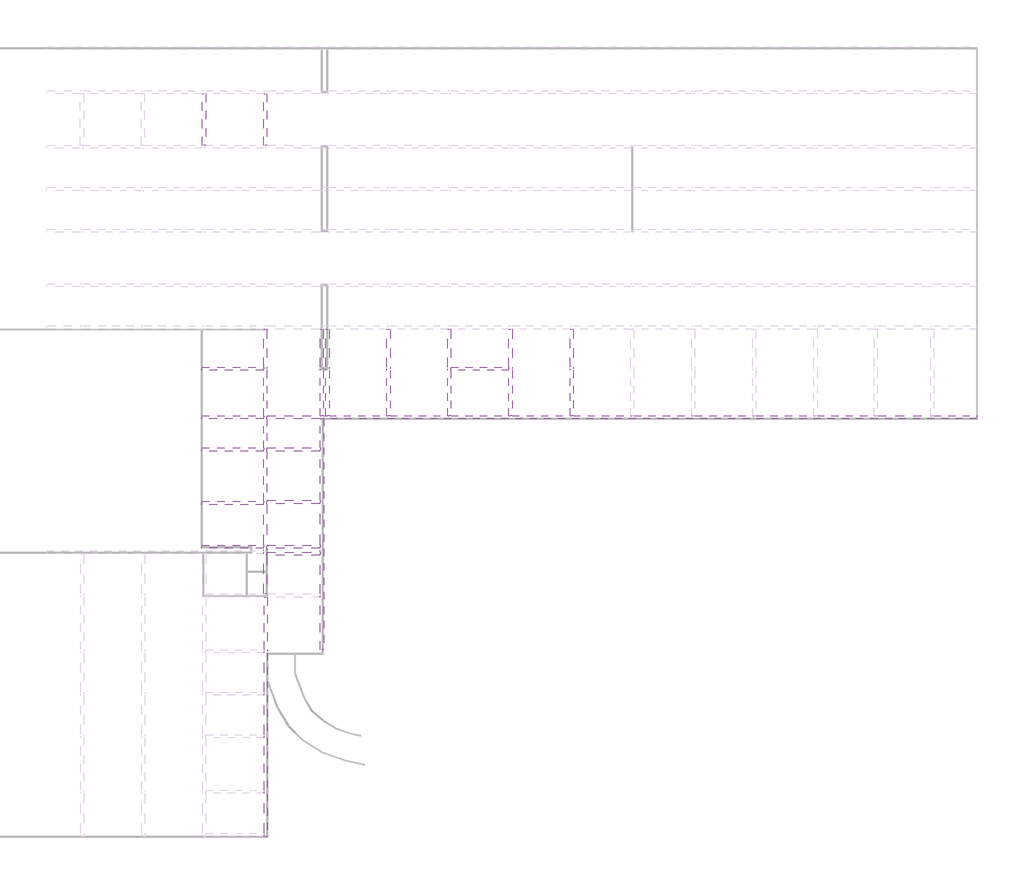
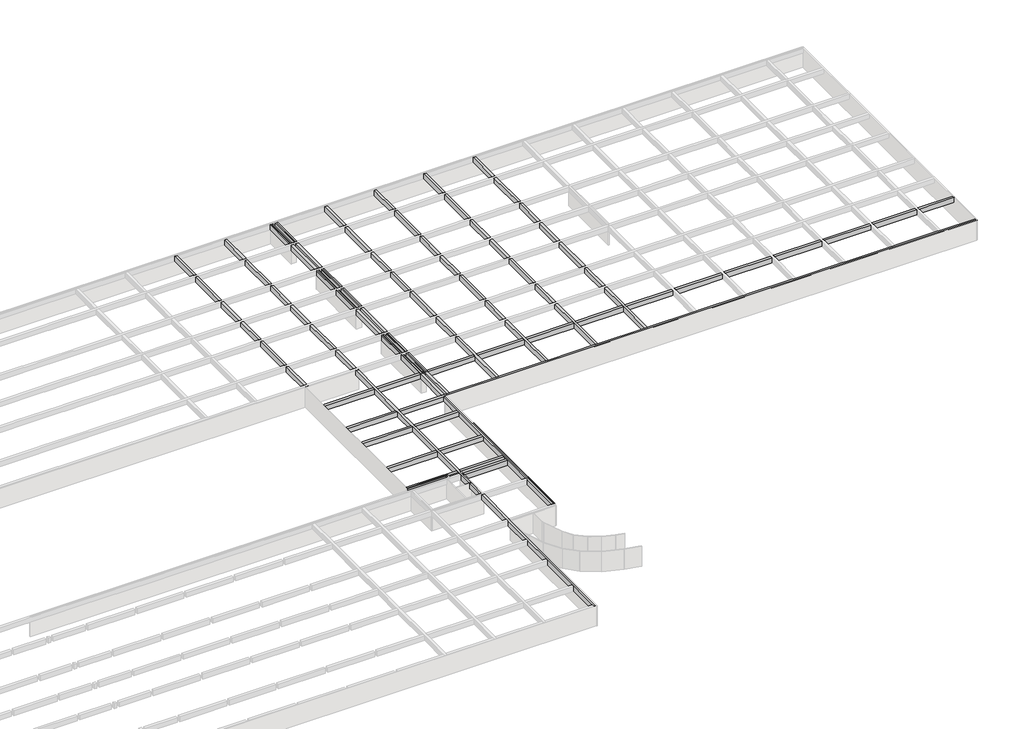
# One storey, part 13 of 14: 22 beams.
"""IFC4 building model written with IfcOpenShell, lengths in millimetres."""

from ifc_helpers import new_model, si_unit, frame, origin, place, context, project, spatial, polyline, outline, extrude, faceted_brep, element, save

model = new_model("IFC4")

# Units and contexts
model_context = context("Model", 3, world=origin())
ifc_project = project(units=[si_unit("LENGTHUNIT", "METRE", prefix="MILLI")], contexts=[model_context])

# Site, building, storey
site = spatial("IfcSite", under=ifc_project)
building = spatial("IfcBuilding", under=site)
storey = spatial("IfcBuildingStorey", under=building, Name="户型图", Elevation=0.0)

# Beams
placement = place(None, origin())
element("IfcBeam", 1, ObjectType="混凝土 - 矩形梁 : KL_beam", at=placement, inside=storey, context=model_context, shape_type="SweptSolid", body=[
    extrude(outline(polyline([(128527.2949044, -153358.950757), (128127.2949044, -153358.950757), (128127.2949044, -153299.284307), (128527.2949044, -153299.284307), (128527.2949044, -153358.950757)])), frame((0.0, 0.0, 2500.0), z_axis=(0.0, 0.0, 1.0), x_axis=(1.0, 0.0, 0.0)), (0.0, 0.0, 1.0), 800.0),
    extrude(outline(polyline([(128527.2949044, -122797.8127788), (128127.2949044, -122797.8127788), (128127.2949044, -117558.950757), (128527.2949044, -117558.950757), (128527.2949044, -122797.8127788)])), frame((0.0, 0.0, 2500.0), z_axis=(0.0, 0.0, 1.0), x_axis=(1.0, 0.0, 0.0)), (0.0, 0.0, 1.0), 800.0),
    extrude(outline(polyline([(128127.2949044, -123197.8127788), (128527.2949044, -123197.8127788), (128527.2949044, -129780.0179086), (128127.2949044, -129780.0179086), (128127.2949044, -123197.8127788)])), frame((0.0, 0.0, 2500.0), z_axis=(0.0, 0.0, 1.0), x_axis=(1.0, 0.0, 0.0)), (0.0, 0.0, 1.0), 800.0),
    extrude(outline(polyline([(128127.2949044, -130180.0179086), (128527.2949044, -130180.0179086), (128527.2949044, -135180.0179086), (128127.2949044, -135180.0179086), (128127.2949044, -130180.0179086)])), frame((0.0, 0.0, 2500.0), z_axis=(0.0, 0.0, 1.0), x_axis=(1.0, 0.0, 0.0)), (0.0, 0.0, 1.0), 800.0),
    extrude(outline(polyline([(128127.2949044, -135580.0179086), (128527.2949044, -135580.0179086), (128527.2949044, -140520.0179086), (128127.2949044, -140520.0179086), (128127.2949044, -135580.0179086)])), frame((0.0, 0.0, 2500.0), z_axis=(0.0, 0.0, 1.0), x_axis=(1.0, 0.0, 0.0)), (0.0, 0.0, 1.0), 800.0),
    extrude(outline(polyline([(128127.2949044, -140920.0179086), (128527.2949044, -140920.0179086), (128527.2949044, -147499.284307), (128127.2949044, -147499.284307), (128127.2949044, -140920.0179086)])), frame((0.0, 0.0, 2500.0), z_axis=(0.0, 0.0, 1.0), x_axis=(1.0, 0.0, 0.0)), (0.0, 0.0, 1.0), 800.0),
    extrude(outline(polyline([(128127.2949044, -147899.284307), (128527.2949044, -147899.284307), (128527.2949044, -152899.284307), (128127.2949044, -152899.284307), (128127.2949044, -147899.284307)])), frame((0.0, 0.0, 2500.0), z_axis=(0.0, 0.0, 1.0), x_axis=(1.0, 0.0, 0.0)), (0.0, 0.0, 1.0), 800.0),
])
element("IfcBeam", 2, ObjectType="混凝土 - 矩形梁 : KL_beam", at=placement, inside=storey, context=model_context, shape_type="SweptSolid", body=[
    extrude(outline(polyline([(136347.2949044, -153358.950757), (135947.2949044, -153358.950757), (135947.2949044, -153299.284307), (136347.2949044, -153299.284307), (136347.2949044, -153358.950757)])), frame((0.0, 0.0, 2500.0), z_axis=(0.0, 0.0, 1.0), x_axis=(1.0, 0.0, 0.0)), (0.0, 0.0, 1.0), 800.0),
    extrude(outline(polyline([(135947.2949044, -123197.8127788), (136347.2949044, -123197.8127788), (136347.2949044, -129780.0179086), (135947.2949044, -129780.0179086), (135947.2949044, -123197.8127788)])), frame((0.0, 0.0, 2500.0), z_axis=(0.0, 0.0, 1.0), x_axis=(1.0, 0.0, 0.0)), (0.0, 0.0, 1.0), 800.0),
    extrude(outline(polyline([(136347.2949044, -122797.8127788), (135947.2949044, -122797.8127788), (135947.2949044, -117558.950757), (136347.2949044, -117558.950757), (136347.2949044, -122797.8127788)])), frame((0.0, 0.0, 2500.0), z_axis=(0.0, 0.0, 1.0), x_axis=(1.0, 0.0, 0.0)), (0.0, 0.0, 1.0), 800.0),
    extrude(outline(polyline([(135947.2949044, -130180.0179086), (136347.2949044, -130180.0179086), (136347.2949044, -135180.0179086), (135947.2949044, -135180.0179086), (135947.2949044, -130180.0179086)])), frame((0.0, 0.0, 2500.0), z_axis=(0.0, 0.0, 1.0), x_axis=(1.0, 0.0, 0.0)), (0.0, 0.0, 1.0), 800.0),
    extrude(outline(polyline([(135947.2949044, -135580.0179086), (136347.2949044, -135580.0179086), (136347.2949044, -140520.0179086), (135947.2949044, -140520.0179086), (135947.2949044, -135580.0179086)])), frame((0.0, 0.0, 2500.0), z_axis=(0.0, 0.0, 1.0), x_axis=(1.0, 0.0, 0.0)), (0.0, 0.0, 1.0), 800.0),
    extrude(outline(polyline([(135947.2949044, -140920.0179086), (136347.2949044, -140920.0179086), (136347.2949044, -147499.284307), (135947.2949044, -147499.284307), (135947.2949044, -140920.0179086)])), frame((0.0, 0.0, 2500.0), z_axis=(0.0, 0.0, 1.0), x_axis=(1.0, 0.0, 0.0)), (0.0, 0.0, 1.0), 800.0),
    extrude(outline(polyline([(135947.2949044, -147899.284307), (136347.2949044, -147899.284307), (136347.2949044, -152899.284307), (135947.2949044, -152899.284307), (135947.2949044, -147899.284307)])), frame((0.0, 0.0, 2500.0), z_axis=(0.0, 0.0, 1.0), x_axis=(1.0, 0.0, 0.0)), (0.0, 0.0, 1.0), 800.0),
])
element("IfcBeam", 3, ObjectType="混凝土 - 矩形梁 : KL_beam", at=placement, inside=storey, context=model_context, shape_type="Brep", body=[
    faceted_brep([(143177.2949044, -122797.8127788, 3300.0), (143577.2949044, -122797.8127788, 3300.0), (143577.2949044, -117558.950757, 3300.0), (143177.2949044, -117558.950757, 3300.0), (143177.2949044, -122797.8127788, 2500.0), (143177.2949044, -117558.950757, 2500.0), (143577.2949044, -122797.8127788, 2500.0), (143577.2949044, -117558.950757, 2500.0)], [[[0, 1, 2, 3]], [[4, 0, 3, 5]], [[6, 4, 5, 7]], [[1, 6, 7, 2]], [[1, 0, 4, 6]], [[3, 2, 7, 5]]]),
    faceted_brep([(143177.2949044, -123197.8127788, 3300.0), (143577.2949044, -123197.8127788, 3300.0), (143577.2949044, -123197.8127788, 2500.0), (143177.2949044, -123197.8127788, 2500.0), (143577.2949044, -129780.0179086, 3300.0), (143177.2949044, -129780.0179086, 3300.0), (143177.2949044, -129780.0179086, 2500.0), (143577.2949044, -129780.0179086, 2500.0)], [[[0, 1, 2, 3]], [[4, 5, 6, 7]], [[1, 0, 5, 4]], [[0, 3, 6, 5]], [[3, 2, 7, 6]], [[2, 1, 4, 7]]]),
    faceted_brep([(143577.2949044, -130180.0179086, 3300.0), (143177.2949044, -130180.0179086, 3300.0), (143177.2949044, -135180.0179086, 3300.0), (143577.2949044, -135180.0179086, 3300.0), (143177.2949044, -130180.0179086, 2500.0), (143177.2949044, -135180.0179086, 2500.0), (143577.2949044, -130180.0179086, 2500.0), (143577.2949044, -135180.0179086, 2500.0)], [[[0, 1, 2, 3]], [[1, 4, 5, 2]], [[4, 6, 7, 5]], [[6, 0, 3, 7]], [[1, 0, 6, 4]], [[3, 2, 5, 7]]]),
    faceted_brep([(143177.2949044, -135580.0179086, 3300.0), (143577.2949044, -135580.0179086, 3300.0), (143577.2949044, -135580.0179086, 2500.0), (143177.2949044, -135580.0179086, 2500.0), (143577.2949044, -140520.0179086, 3300.0), (143177.2949044, -140520.0179086, 3300.0), (143177.2949044, -140520.0179086, 2500.0), (143577.2949044, -140520.0179086, 2500.0)], [[[0, 1, 2, 3]], [[4, 5, 6, 7]], [[1, 0, 5, 4]], [[0, 3, 6, 5]], [[3, 2, 7, 6]], [[2, 1, 4, 7]]]),
    faceted_brep([(143177.2949044, -140920.0179086, 3300.0), (143577.2949044, -140920.0179086, 3300.0), (143577.2949044, -140920.0179086, 2500.0), (143177.2949044, -140920.0179086, 2500.0), (143577.2949044, -147499.284307, 3300.0), (143177.2949044, -147499.284307, 3300.0), (143177.2949044, -147499.284307, 2500.0), (143577.2949044, -147499.284307, 2500.0)], [[[0, 1, 2, 3]], [[4, 5, 6, 7]], [[1, 0, 5, 4]], [[0, 3, 6, 5]], [[3, 2, 7, 6]], [[2, 1, 4, 7]]]),
    faceted_brep([(143177.2949044, -147899.284307, 3300.0), (143577.2949044, -147899.284307, 3300.0), (143577.2949044, -147899.284307, 2500.0), (143177.2949044, -147899.284307, 2500.0), (143577.2949044, -152899.284307, 3300.0), (143177.2949044, -152899.284307, 3300.0), (143177.2949044, -152899.284307, 2500.0), (143577.2949044, -152899.284307, 2500.0)], [[[0, 1, 2, 3]], [[4, 5, 6, 7]], [[1, 0, 5, 4]], [[0, 3, 6, 5]], [[3, 2, 7, 6]], [[2, 1, 4, 7]]]),
    faceted_brep([(143177.2949044, -153299.284307, 3300.0), (143577.2949044, -153299.284307, 3300.0), (143577.2949044, -153299.284307, 2500.0), (143177.2949044, -153299.284307, 2500.0), (143577.2949044, -164396.0449275, 3300.0), (143177.2949044, -164396.0449275, 3300.0), (143177.2949044, -164396.0449275, 2500.0), (143577.2949044, -164396.0449275, 2500.0), (143177.2949044, -158198.950757, 3300.0), (143177.2949044, -158598.950757, 3300.0), (143577.2949044, -158598.950757, 3300.0), (143577.2949044, -158198.950757, 3300.0), (143177.2949044, -158198.950757, 2500.0), (143177.2949044, -158598.950757, 2500.0), (143577.2949044, -158198.950757, 2500.0), (143577.2949044, -158598.950757, 2500.0)], [[[0, 1, 2, 3]], [[4, 5, 6, 7]], [[1, 0, 8, 9, 5, 4, 10, 11]], [[0, 3, 12, 13, 6, 5, 9, 8]], [[3, 2, 14, 15, 7, 6, 13, 12]], [[2, 1, 11, 10, 4, 7, 15, 14]]]),
])
element("IfcBeam", 4, ObjectType="混凝土 - 矩形梁 : KL_beam", at=placement, inside=storey, context=model_context, shape_type="Brep", body=[
    faceted_brep([(144337.2949044, -153299.284307, 3300.0), (143937.2949044, -153299.284307, 3300.0), (143937.2949044, -158198.950757, 3300.0), (143937.2949044, -158598.950757, 3300.0), (143937.2949044, -164396.0449275, 3300.0), (144337.2949044, -164396.0449275, 3300.0), (144337.2949044, -158598.950757, 3300.0), (144337.2949044, -158198.950757, 3300.0), (144337.2949044, -153299.284307, 2500.0), (144337.2949044, -164396.0449275, 2500.0), (144337.2949044, -158598.950757, 2500.0), (144337.2949044, -158198.950757, 2500.0), (143937.2949044, -153299.284307, 2500.0), (143937.2949044, -164396.0449275, 2500.0), (143937.2949044, -158598.950757, 2500.0), (143937.2949044, -158198.950757, 2500.0)], [[[0, 1, 2, 3, 4, 5, 6, 7]], [[8, 0, 7, 6, 5, 9, 10, 11]], [[12, 8, 11, 10, 9, 13, 14, 15]], [[1, 12, 15, 14, 13, 4, 3, 2]], [[1, 0, 8, 12]], [[5, 4, 13, 9]]]),
    faceted_brep([(143937.2949044, -123197.8127788, 3300.0), (144337.2949044, -123197.8127788, 3300.0), (144337.2949044, -123197.8127788, 2500.0), (143937.2949044, -123197.8127788, 2500.0), (144337.2949044, -129780.0179086, 3300.0), (143937.2949044, -129780.0179086, 3300.0), (143937.2949044, -129780.0179086, 2500.0), (144337.2949044, -129780.0179086, 2500.0)], [[[0, 1, 2, 3]], [[4, 5, 6, 7]], [[1, 0, 5, 4]], [[2, 1, 4, 7]], [[3, 2, 7, 6]], [[0, 3, 6, 5]]]),
    faceted_brep([(144337.2949044, -122797.8127788, 3300.0), (143937.2949044, -122797.8127788, 3300.0), (143937.2949044, -122797.8127788, 2500.0), (144337.2949044, -122797.8127788, 2500.0), (144337.2949044, -117558.950757, 3300.0), (143937.2949044, -117558.950757, 3300.0), (144337.2949044, -117558.950757, 2500.0), (143937.2949044, -117558.950757, 2500.0)], [[[0, 1, 2, 3]], [[1, 0, 4, 5]], [[0, 3, 6, 4]], [[3, 2, 7, 6]], [[2, 1, 5, 7]], [[5, 4, 6, 7]]]),
    faceted_brep([(143937.2949044, -130180.0179086, 3300.0), (144337.2949044, -130180.0179086, 3300.0), (144337.2949044, -130180.0179086, 2500.0), (143937.2949044, -130180.0179086, 2500.0), (144337.2949044, -135180.0179086, 3300.0), (143937.2949044, -135180.0179086, 3300.0), (143937.2949044, -135180.0179086, 2500.0), (144337.2949044, -135180.0179086, 2500.0)], [[[0, 1, 2, 3]], [[4, 5, 6, 7]], [[1, 0, 5, 4]], [[2, 1, 4, 7]], [[3, 2, 7, 6]], [[0, 3, 6, 5]]]),
    faceted_brep([(143937.2949044, -135580.0179086, 3300.0), (144337.2949044, -135580.0179086, 3300.0), (144337.2949044, -135580.0179086, 2500.0), (143937.2949044, -135580.0179086, 2500.0), (144337.2949044, -140520.0179086, 3300.0), (143937.2949044, -140520.0179086, 3300.0), (143937.2949044, -140520.0179086, 2500.0), (144337.2949044, -140520.0179086, 2500.0)], [[[0, 1, 2, 3]], [[4, 5, 6, 7]], [[1, 0, 5, 4]], [[2, 1, 4, 7]], [[3, 2, 7, 6]], [[0, 3, 6, 5]]]),
    faceted_brep([(143937.2949044, -140920.0179086, 3300.0), (144337.2949044, -140920.0179086, 3300.0), (144337.2949044, -140920.0179086, 2500.0), (143937.2949044, -140920.0179086, 2500.0), (144337.2949044, -147499.284307, 3300.0), (143937.2949044, -147499.284307, 3300.0), (143937.2949044, -147499.284307, 2500.0), (144337.2949044, -147499.284307, 2500.0)], [[[0, 1, 2, 3]], [[4, 5, 6, 7]], [[1, 0, 5, 4]], [[2, 1, 4, 7]], [[3, 2, 7, 6]], [[0, 3, 6, 5]]]),
    faceted_brep([(143937.2949044, -147899.284307, 3300.0), (144337.2949044, -147899.284307, 3300.0), (144337.2949044, -147899.284307, 2500.0), (143937.2949044, -147899.284307, 2500.0), (144337.2949044, -152899.284307, 3300.0), (143937.2949044, -152899.284307, 3300.0), (143937.2949044, -152899.284307, 2500.0), (144337.2949044, -152899.284307, 2500.0)], [[[0, 1, 2, 3]], [[4, 5, 6, 7]], [[1, 0, 5, 4]], [[2, 1, 4, 7]], [[3, 2, 7, 6]], [[0, 3, 6, 5]]]),
])
element("IfcBeam", 5, ObjectType="混凝土 - 矩形梁 : KL_beam", at=placement, inside=storey, context=model_context, shape_type="Brep", body=[
    faceted_brep([(151740.9658811, -122797.8127788, 3300.0), (152140.9658811, -122797.8127788, 3300.0), (152140.9658811, -117558.950757, 3300.0), (151740.9658811, -117558.950757, 3300.0), (151740.9658811, -122797.8127788, 2500.0), (151740.9658811, -117558.950757, 2500.0), (152140.9658811, -122797.8127788, 2500.0), (152140.9658811, -117558.950757, 2500.0)], [[[0, 1, 2, 3]], [[4, 0, 3, 5]], [[6, 4, 5, 7]], [[1, 6, 7, 2]], [[1, 0, 4, 6]], [[3, 2, 7, 5]]]),
    faceted_brep([(151740.9658811, -123197.8127788, 3300.0), (152140.9658811, -123197.8127788, 3300.0), (152140.9658811, -123197.8127788, 2500.0), (151740.9658811, -123197.8127788, 2500.0), (152140.9658811, -129780.0179086, 3300.0), (151740.9658811, -129780.0179086, 3300.0), (151740.9658811, -129780.0179086, 2500.0), (152140.9658811, -129780.0179086, 2500.0)], [[[0, 1, 2, 3]], [[4, 5, 6, 7]], [[1, 0, 5, 4]], [[0, 3, 6, 5]], [[3, 2, 7, 6]], [[2, 1, 4, 7]]]),
    faceted_brep([(152140.9658811, -130180.0179086, 3300.0), (151740.9658811, -130180.0179086, 3300.0), (151740.9658811, -135180.0179086, 3300.0), (152140.9658811, -135180.0179086, 3300.0), (151740.9658811, -130180.0179086, 2500.0), (151740.9658811, -135180.0179086, 2500.0), (152140.9658811, -130180.0179086, 2500.0), (152140.9658811, -135180.0179086, 2500.0)], [[[0, 1, 2, 3]], [[1, 4, 5, 2]], [[4, 6, 7, 5]], [[6, 0, 3, 7]], [[1, 0, 6, 4]], [[3, 2, 5, 7]]]),
    faceted_brep([(151740.9658811, -135580.0179086, 3300.0), (152140.9658811, -135580.0179086, 3300.0), (152140.9658811, -135580.0179086, 2500.0), (151740.9658811, -135580.0179086, 2500.0), (152140.9658811, -140520.0179086, 3300.0), (151740.9658811, -140520.0179086, 3300.0), (151740.9658811, -140520.0179086, 2500.0), (152140.9658811, -140520.0179086, 2500.0)], [[[0, 1, 2, 3]], [[4, 5, 6, 7]], [[1, 0, 5, 4]], [[0, 3, 6, 5]], [[3, 2, 7, 6]], [[2, 1, 4, 7]]]),
    faceted_brep([(151740.9658811, -140920.0179086, 3300.0), (152140.9658811, -140920.0179086, 3300.0), (152140.9658811, -140920.0179086, 2500.0), (151740.9658811, -140920.0179086, 2500.0), (152140.9658811, -147499.284307, 3300.0), (151740.9658811, -147499.284307, 3300.0), (151740.9658811, -147499.284307, 2500.0), (152140.9658811, -147499.284307, 2500.0)], [[[0, 1, 2, 3]], [[4, 5, 6, 7]], [[1, 0, 5, 4]], [[0, 3, 6, 5]], [[3, 2, 7, 6]], [[2, 1, 4, 7]]]),
    faceted_brep([(151740.9658811, -147899.284307, 3300.0), (152140.9658811, -147899.284307, 3300.0), (152140.9658811, -147899.284307, 2500.0), (151740.9658811, -147899.284307, 2500.0), (152140.9658811, -152899.284307, 3300.0), (151740.9658811, -152899.284307, 3300.0), (151740.9658811, -152899.284307, 2500.0), (152140.9658811, -152899.284307, 2500.0)], [[[0, 1, 2, 3]], [[4, 5, 6, 7]], [[1, 0, 5, 4]], [[0, 3, 6, 5]], [[3, 2, 7, 6]], [[2, 1, 4, 7]]]),
    faceted_brep([(151740.9658811, -153299.284307, 3300.0), (152140.9658811, -153299.284307, 3300.0), (152140.9658811, -153299.284307, 2500.0), (151740.9658811, -153299.284307, 2500.0), (152140.9658811, -164396.0449275, 3300.0), (151740.9658811, -164396.0449275, 3300.0), (151740.9658811, -164396.0449275, 2500.0), (152140.9658811, -164396.0449275, 2500.0), (151740.9658811, -158198.950757, 3300.0), (151740.9658811, -158598.950757, 3300.0), (152140.9658811, -158598.950757, 3300.0), (152140.9658811, -158198.950757, 3300.0), (151740.9658811, -158198.950757, 2500.0), (151740.9658811, -158598.950757, 2500.0), (152140.9658811, -158198.950757, 2500.0), (152140.9658811, -158598.950757, 2500.0)], [[[0, 1, 2, 3]], [[4, 5, 6, 7]], [[1, 0, 8, 9, 5, 4, 10, 11]], [[0, 3, 12, 13, 6, 5, 9, 8]], [[3, 2, 14, 15, 7, 6, 13, 12]], [[2, 1, 11, 10, 4, 7, 15, 14]]]),
])
element("IfcBeam", 6, ObjectType="混凝土 - 矩形梁 : KL_beam", at=placement, inside=storey, context=model_context, shape_type="Brep", body=[
    faceted_brep([(159907.8874304, -153299.284307, 3300.0), (159507.8874304, -153299.284307, 3300.0), (159507.8874304, -158198.950757, 3300.0), (159507.8874304, -158598.950757, 3300.0), (159507.8874304, -164396.0449275, 3300.0), (159907.8874304, -164396.0449275, 3300.0), (159907.8874304, -158598.950757, 3300.0), (159907.8874304, -158198.950757, 3300.0), (159907.8874304, -153299.284307, 2500.0), (159907.8874304, -164396.0449275, 2500.0), (159907.8874304, -158598.950757, 2500.0), (159907.8874304, -158198.950757, 2500.0), (159507.8874304, -153299.284307, 2500.0), (159507.8874304, -164396.0449275, 2500.0), (159507.8874304, -158598.950757, 2500.0), (159507.8874304, -158198.950757, 2500.0)], [[[0, 1, 2, 3, 4, 5, 6, 7]], [[8, 0, 7, 6, 5, 9, 10, 11]], [[12, 8, 11, 10, 9, 13, 14, 15]], [[1, 12, 15, 14, 13, 4, 3, 2]], [[1, 0, 8, 12]], [[5, 4, 13, 9]]]),
    faceted_brep([(159507.8874304, -123197.8127788, 3300.0), (159907.8874304, -123197.8127788, 3300.0), (159907.8874304, -123197.8127788, 2500.0), (159507.8874304, -123197.8127788, 2500.0), (159907.8874304, -129780.0179086, 3300.0), (159507.8874304, -129780.0179086, 3300.0), (159507.8874304, -129780.0179086, 2500.0), (159907.8874304, -129780.0179086, 2500.0)], [[[0, 1, 2, 3]], [[4, 5, 6, 7]], [[1, 0, 5, 4]], [[2, 1, 4, 7]], [[3, 2, 7, 6]], [[0, 3, 6, 5]]]),
    faceted_brep([(159907.8874304, -122797.8127788, 3300.0), (159507.8874304, -122797.8127788, 3300.0), (159507.8874304, -122797.8127788, 2500.0), (159907.8874304, -122797.8127788, 2500.0), (159907.8874304, -117558.950757, 3300.0), (159507.8874304, -117558.950757, 3300.0), (159907.8874304, -117558.950757, 2500.0), (159507.8874304, -117558.950757, 2500.0)], [[[0, 1, 2, 3]], [[1, 0, 4, 5]], [[0, 3, 6, 4]], [[3, 2, 7, 6]], [[2, 1, 5, 7]], [[5, 4, 6, 7]]]),
    faceted_brep([(159507.8874304, -130180.0179086, 3300.0), (159907.8874304, -130180.0179086, 3300.0), (159907.8874304, -130180.0179086, 2500.0), (159507.8874304, -130180.0179086, 2500.0), (159907.8874304, -135180.0179086, 3300.0), (159507.8874304, -135180.0179086, 3300.0), (159507.8874304, -135180.0179086, 2500.0), (159907.8874304, -135180.0179086, 2500.0)], [[[0, 1, 2, 3]], [[4, 5, 6, 7]], [[1, 0, 5, 4]], [[2, 1, 4, 7]], [[3, 2, 7, 6]], [[0, 3, 6, 5]]]),
    faceted_brep([(159507.8874304, -135580.0179086, 3300.0), (159907.8874304, -135580.0179086, 3300.0), (159907.8874304, -135580.0179086, 2500.0), (159507.8874304, -135580.0179086, 2500.0), (159907.8874304, -140520.0179086, 3300.0), (159507.8874304, -140520.0179086, 3300.0), (159507.8874304, -140520.0179086, 2500.0), (159907.8874304, -140520.0179086, 2500.0)], [[[0, 1, 2, 3]], [[4, 5, 6, 7]], [[1, 0, 5, 4]], [[2, 1, 4, 7]], [[3, 2, 7, 6]], [[0, 3, 6, 5]]]),
    faceted_brep([(159507.8874304, -140920.0179086, 3300.0), (159907.8874304, -140920.0179086, 3300.0), (159907.8874304, -140920.0179086, 2500.0), (159507.8874304, -140920.0179086, 2500.0), (159907.8874304, -147499.284307, 3300.0), (159507.8874304, -147499.284307, 3300.0), (159507.8874304, -147499.284307, 2500.0), (159907.8874304, -147499.284307, 2500.0)], [[[0, 1, 2, 3]], [[4, 5, 6, 7]], [[1, 0, 5, 4]], [[2, 1, 4, 7]], [[3, 2, 7, 6]], [[0, 3, 6, 5]]]),
    faceted_brep([(159507.8874304, -147899.284307, 3300.0), (159907.8874304, -147899.284307, 3300.0), (159907.8874304, -147899.284307, 2500.0), (159507.8874304, -147899.284307, 2500.0), (159907.8874304, -152899.284307, 3300.0), (159507.8874304, -152899.284307, 3300.0), (159507.8874304, -152899.284307, 2500.0), (159907.8874304, -152899.284307, 2500.0)], [[[0, 1, 2, 3]], [[4, 5, 6, 7]], [[1, 0, 5, 4]], [[2, 1, 4, 7]], [[3, 2, 7, 6]], [[0, 3, 6, 5]]]),
])
element("IfcBeam", 7, ObjectType="混凝土 - 矩形梁 : KL_beam", at=placement, inside=storey, context=model_context, shape_type="Brep", body=[
    faceted_brep([(167340.9658811, -122797.8127788, 3300.0), (167740.9658811, -122797.8127788, 3300.0), (167740.9658811, -117558.950757, 3300.0), (167340.9658811, -117558.950757, 3300.0), (167340.9658811, -122797.8127788, 2500.0), (167340.9658811, -117558.950757, 2500.0), (167740.9658811, -122797.8127788, 2500.0), (167740.9658811, -117558.950757, 2500.0)], [[[0, 1, 2, 3]], [[4, 0, 3, 5]], [[6, 4, 5, 7]], [[1, 6, 7, 2]], [[1, 0, 4, 6]], [[3, 2, 7, 5]]]),
    faceted_brep([(167340.9658811, -123197.8127788, 3300.0), (167740.9658811, -123197.8127788, 3300.0), (167740.9658811, -123197.8127788, 2500.0), (167340.9658811, -123197.8127788, 2500.0), (167740.9658811, -129780.0179086, 3300.0), (167340.9658811, -129780.0179086, 3300.0), (167340.9658811, -129780.0179086, 2500.0), (167740.9658811, -129780.0179086, 2500.0)], [[[0, 1, 2, 3]], [[4, 5, 6, 7]], [[1, 0, 5, 4]], [[0, 3, 6, 5]], [[3, 2, 7, 6]], [[2, 1, 4, 7]]]),
    faceted_brep([(167740.9658811, -130180.0179086, 3300.0), (167340.9658811, -130180.0179086, 3300.0), (167340.9658811, -135180.0179086, 3300.0), (167740.9658811, -135180.0179086, 3300.0), (167340.9658811, -130180.0179086, 2500.0), (167340.9658811, -135180.0179086, 2500.0), (167740.9658811, -130180.0179086, 2500.0), (167740.9658811, -135180.0179086, 2500.0)], [[[0, 1, 2, 3]], [[1, 4, 5, 2]], [[4, 6, 7, 5]], [[6, 0, 3, 7]], [[1, 0, 6, 4]], [[3, 2, 5, 7]]]),
    faceted_brep([(167340.9658811, -135580.0179086, 3300.0), (167740.9658811, -135580.0179086, 3300.0), (167740.9658811, -135580.0179086, 2500.0), (167340.9658811, -135580.0179086, 2500.0), (167740.9658811, -140520.0179086, 3300.0), (167340.9658811, -140520.0179086, 3300.0), (167340.9658811, -140520.0179086, 2500.0), (167740.9658811, -140520.0179086, 2500.0)], [[[0, 1, 2, 3]], [[4, 5, 6, 7]], [[1, 0, 5, 4]], [[0, 3, 6, 5]], [[3, 2, 7, 6]], [[2, 1, 4, 7]]]),
    faceted_brep([(167340.9658811, -140920.0179086, 3300.0), (167740.9658811, -140920.0179086, 3300.0), (167740.9658811, -140920.0179086, 2500.0), (167340.9658811, -140920.0179086, 2500.0), (167740.9658811, -147499.284307, 3300.0), (167340.9658811, -147499.284307, 3300.0), (167340.9658811, -147499.284307, 2500.0), (167740.9658811, -147499.284307, 2500.0)], [[[0, 1, 2, 3]], [[4, 5, 6, 7]], [[1, 0, 5, 4]], [[0, 3, 6, 5]], [[3, 2, 7, 6]], [[2, 1, 4, 7]]]),
    faceted_brep([(167340.9658811, -147899.284307, 3300.0), (167740.9658811, -147899.284307, 3300.0), (167740.9658811, -147899.284307, 2500.0), (167340.9658811, -147899.284307, 2500.0), (167740.9658811, -152899.284307, 3300.0), (167340.9658811, -152899.284307, 3300.0), (167340.9658811, -152899.284307, 2500.0), (167740.9658811, -152899.284307, 2500.0)], [[[0, 1, 2, 3]], [[4, 5, 6, 7]], [[1, 0, 5, 4]], [[0, 3, 6, 5]], [[3, 2, 7, 6]], [[2, 1, 4, 7]]]),
    faceted_brep([(167340.9658811, -153299.284307, 3300.0), (167740.9658811, -153299.284307, 3300.0), (167740.9658811, -153299.284307, 2500.0), (167340.9658811, -153299.284307, 2500.0), (167740.9658811, -164396.0449275, 3300.0), (167340.9658811, -164396.0449275, 3300.0), (167340.9658811, -164396.0449275, 2500.0), (167740.9658811, -164396.0449275, 2500.0), (167340.9658811, -158198.950757, 3300.0), (167340.9658811, -158598.950757, 3300.0), (167740.9658811, -158598.950757, 3300.0), (167740.9658811, -158198.950757, 3300.0), (167340.9658811, -158198.950757, 2500.0), (167340.9658811, -158598.950757, 2500.0), (167740.9658811, -158198.950757, 2500.0), (167740.9658811, -158598.950757, 2500.0)], [[[0, 1, 2, 3]], [[4, 5, 6, 7]], [[1, 0, 8, 9, 5, 4, 10, 11]], [[0, 3, 12, 13, 6, 5, 9, 8]], [[3, 2, 14, 15, 7, 6, 13, 12]], [[2, 1, 11, 10, 4, 7, 15, 14]]]),
])
element("IfcBeam", 8, ObjectType="混凝土 - 矩形梁 : KL_beam", at=placement, inside=storey, context=model_context, shape_type="Brep", body=[
    faceted_brep([(175558.5232577, -153299.284307, 3300.0), (175158.5232577, -153299.284307, 3300.0), (175158.5232577, -158198.950757, 3300.0), (175158.5232577, -158598.950757, 3300.0), (175158.5232577, -164396.0449275, 3300.0), (175558.5232577, -164396.0449275, 3300.0), (175558.5232577, -158598.950757, 3300.0), (175558.5232577, -158198.950757, 3300.0), (175558.5232577, -153299.284307, 2500.0), (175558.5232577, -164396.0449275, 2500.0), (175558.5232577, -158598.950757, 2500.0), (175558.5232577, -158198.950757, 2500.0), (175158.5232577, -153299.284307, 2500.0), (175158.5232577, -164396.0449275, 2500.0), (175158.5232577, -158598.950757, 2500.0), (175158.5232577, -158198.950757, 2500.0)], [[[0, 1, 2, 3, 4, 5, 6, 7]], [[8, 0, 7, 6, 5, 9, 10, 11]], [[12, 8, 11, 10, 9, 13, 14, 15]], [[1, 12, 15, 14, 13, 4, 3, 2]], [[1, 0, 8, 12]], [[5, 4, 13, 9]]]),
    faceted_brep([(175158.5232577, -123197.8127788, 3300.0), (175558.5232577, -123197.8127788, 3300.0), (175558.5232577, -123197.8127788, 2500.0), (175158.5232577, -123197.8127788, 2500.0), (175558.5232577, -129780.0179086, 3300.0), (175158.5232577, -129780.0179086, 3300.0), (175158.5232577, -129780.0179086, 2500.0), (175558.5232577, -129780.0179086, 2500.0)], [[[0, 1, 2, 3]], [[4, 5, 6, 7]], [[1, 0, 5, 4]], [[2, 1, 4, 7]], [[3, 2, 7, 6]], [[0, 3, 6, 5]]]),
    faceted_brep([(175558.5232577, -122797.8127788, 3300.0), (175158.5232577, -122797.8127788, 3300.0), (175158.5232577, -122797.8127788, 2500.0), (175558.5232577, -122797.8127788, 2500.0), (175558.5232577, -117558.950757, 3300.0), (175158.5232577, -117558.950757, 3300.0), (175558.5232577, -117558.950757, 2500.0), (175158.5232577, -117558.950757, 2500.0)], [[[0, 1, 2, 3]], [[1, 0, 4, 5]], [[0, 3, 6, 4]], [[3, 2, 7, 6]], [[2, 1, 5, 7]], [[5, 4, 6, 7]]]),
    faceted_brep([(175158.5232577, -130180.0179086, 3300.0), (175558.5232577, -130180.0179086, 3300.0), (175558.5232577, -130180.0179086, 2500.0), (175158.5232577, -130180.0179086, 2500.0), (175558.5232577, -135180.0179086, 3300.0), (175158.5232577, -135180.0179086, 3300.0), (175158.5232577, -135180.0179086, 2500.0), (175558.5232577, -135180.0179086, 2500.0)], [[[0, 1, 2, 3]], [[4, 5, 6, 7]], [[1, 0, 5, 4]], [[2, 1, 4, 7]], [[3, 2, 7, 6]], [[0, 3, 6, 5]]]),
    faceted_brep([(175158.5232577, -135580.0179086, 3300.0), (175558.5232577, -135580.0179086, 3300.0), (175558.5232577, -135580.0179086, 2500.0), (175158.5232577, -135580.0179086, 2500.0), (175558.5232577, -140520.0179086, 3300.0), (175158.5232577, -140520.0179086, 3300.0), (175158.5232577, -140520.0179086, 2500.0), (175558.5232577, -140520.0179086, 2500.0)], [[[0, 1, 2, 3]], [[4, 5, 6, 7]], [[1, 0, 5, 4]], [[2, 1, 4, 7]], [[3, 2, 7, 6]], [[0, 3, 6, 5]]]),
    faceted_brep([(175158.5232577, -140920.0179086, 3300.0), (175558.5232577, -140920.0179086, 3300.0), (175558.5232577, -140920.0179086, 2500.0), (175158.5232577, -140920.0179086, 2500.0), (175558.5232577, -147499.284307, 3300.0), (175158.5232577, -147499.284307, 3300.0), (175158.5232577, -147499.284307, 2500.0), (175558.5232577, -147499.284307, 2500.0)], [[[0, 1, 2, 3]], [[4, 5, 6, 7]], [[1, 0, 5, 4]], [[2, 1, 4, 7]], [[3, 2, 7, 6]], [[0, 3, 6, 5]]]),
    faceted_brep([(175158.5232577, -147899.284307, 3300.0), (175558.5232577, -147899.284307, 3300.0), (175558.5232577, -147899.284307, 2500.0), (175158.5232577, -147899.284307, 2500.0), (175558.5232577, -152899.284307, 3300.0), (175158.5232577, -152899.284307, 3300.0), (175158.5232577, -152899.284307, 2500.0), (175558.5232577, -152899.284307, 2500.0)], [[[0, 1, 2, 3]], [[4, 5, 6, 7]], [[1, 0, 5, 4]], [[2, 1, 4, 7]], [[3, 2, 7, 6]], [[0, 3, 6, 5]]]),
])
element("IfcBeam", 9, ObjectType="混凝土 - 矩形梁 : KL_beam", at=placement, inside=storey, context=model_context, shape_type="SweptSolid", body=[
    extrude(outline(polyline([(227227.2949044, -158198.950757), (227227.2949044, -158598.950757), (221727.2949044, -158598.950757), (221727.2949044, -158198.950757), (227227.2949044, -158198.950757)])), frame((0.0, 0.0, 2500.0), z_axis=(0.0, 0.0, 1.0), x_axis=(1.0, 0.0, 0.0)), (0.0, 0.0, 1.0), 800.0),
    extrude(outline(polyline([(143177.2949044, -158198.950757), (143177.2949044, -158598.950757), (136347.2949044, -158598.950757), (136347.2949044, -158198.950757), (143177.2949044, -158198.950757)])), frame((0.0, 0.0, 2500.0), z_axis=(0.0, 0.0, 1.0), x_axis=(1.0, 0.0, 0.0)), (0.0, 0.0, 1.0), 800.0),
    extrude(outline(polyline([(143577.2949044, -158598.950757), (143577.2949044, -158198.950757), (143937.2949044, -158198.950757), (143937.2949044, -158598.950757), (143577.2949044, -158598.950757)])), frame((0.0, 0.0, 2500.0), z_axis=(0.0, 0.0, 1.0), x_axis=(1.0, 0.0, 0.0)), (0.0, 0.0, 1.0), 800.0),
    extrude(outline(polyline([(144337.2949044, -158598.950757), (144337.2949044, -158198.950757), (151740.9658811, -158198.950757), (151740.9658811, -158598.950757), (144337.2949044, -158598.950757)])), frame((0.0, 0.0, 2500.0), z_axis=(0.0, 0.0, 1.0), x_axis=(1.0, 0.0, 0.0)), (0.0, 0.0, 1.0), 800.0),
    extrude(outline(polyline([(152140.9658811, -158598.950757), (152140.9658811, -158198.950757), (159507.8874304, -158198.950757), (159507.8874304, -158598.950757), (152140.9658811, -158598.950757)])), frame((0.0, 0.0, 2500.0), z_axis=(0.0, 0.0, 1.0), x_axis=(1.0, 0.0, 0.0)), (0.0, 0.0, 1.0), 800.0),
    extrude(outline(polyline([(159907.8874304, -158598.950757), (159907.8874304, -158198.950757), (167340.9658811, -158198.950757), (167340.9658811, -158598.950757), (159907.8874304, -158598.950757)])), frame((0.0, 0.0, 2500.0), z_axis=(0.0, 0.0, 1.0), x_axis=(1.0, 0.0, 0.0)), (0.0, 0.0, 1.0), 800.0),
    extrude(outline(polyline([(167740.9658811, -158598.950757), (167740.9658811, -158198.950757), (175158.5232577, -158198.950757), (175158.5232577, -158598.950757), (167740.9658811, -158598.950757)])), frame((0.0, 0.0, 2500.0), z_axis=(0.0, 0.0, 1.0), x_axis=(1.0, 0.0, 0.0)), (0.0, 0.0, 1.0), 800.0),
    extrude(outline(polyline([(175558.5232577, -158598.950757), (175558.5232577, -158198.950757), (182927.7006088, -158198.950757), (182927.7006088, -158598.950757), (175558.5232577, -158598.950757)])), frame((0.0, 0.0, 2500.0), z_axis=(0.0, 0.0, 1.0), x_axis=(1.0, 0.0, 0.0)), (0.0, 0.0, 1.0), 800.0),
    extrude(outline(polyline([(183327.7006088, -158598.950757), (183327.7006088, -158198.950757), (190737.2949044, -158198.950757), (190737.2949044, -158598.950757), (183327.7006088, -158598.950757)])), frame((0.0, 0.0, 2500.0), z_axis=(0.0, 0.0, 1.0), x_axis=(1.0, 0.0, 0.0)), (0.0, 0.0, 1.0), 800.0),
    extrude(outline(polyline([(191137.2949044, -158598.950757), (191137.2949044, -158198.950757), (198549.6658892, -158198.950757), (198549.6658892, -158598.950757), (191137.2949044, -158598.950757)])), frame((0.0, 0.0, 2500.0), z_axis=(0.0, 0.0, 1.0), x_axis=(1.0, 0.0, 0.0)), (0.0, 0.0, 1.0), 800.0),
    extrude(outline(polyline([(198949.6658892, -158598.950757), (198949.6658892, -158198.950757), (206363.3308695, -158198.950757), (206363.3308695, -158598.950757), (198949.6658892, -158598.950757)])), frame((0.0, 0.0, 2500.0), z_axis=(0.0, 0.0, 1.0), x_axis=(1.0, 0.0, 0.0)), (0.0, 0.0, 1.0), 800.0),
    extrude(outline(polyline([(206763.3308695, -158598.950757), (206763.3308695, -158198.950757), (214091.1566028, -158198.950757), (214091.1566028, -158598.950757), (206763.3308695, -158598.950757)])), frame((0.0, 0.0, 2500.0), z_axis=(0.0, 0.0, 1.0), x_axis=(1.0, 0.0, 0.0)), (0.0, 0.0, 1.0), 800.0),
    extrude(outline(polyline([(214491.1566028, -158598.950757), (214491.1566028, -158198.950757), (221327.2949044, -158198.950757), (221327.2949044, -158598.950757), (214491.1566028, -158598.950757)])), frame((0.0, 0.0, 2500.0), z_axis=(0.0, 0.0, 1.0), x_axis=(1.0, 0.0, 0.0)), (0.0, 0.0, 1.0), 800.0),
])
element("IfcBeam", 10, ObjectType="混凝土 - 矩形梁 : KL_beam", at=placement, inside=storey, context=model_context, shape_type="Brep", body=[
    faceted_brep([(136347.2949044, -153358.950757, 3300.0), (135947.2949044, -153358.950757, 3300.0), (135947.2949044, -158198.950757, 3300.0), (135947.2949044, -158598.950757, 3300.0), (135947.2949044, -164396.0449275, 3300.0), (135947.2949044, -164796.0449275, 3300.0), (135947.2949044, -168516.0449275, 3300.0), (135947.2949044, -168916.0449275, 3300.0), (135947.2949044, -175355.5769678, 3300.0), (135947.2949044, -175755.5769678, 3300.0), (135947.2949044, -180948.950757, 3300.0), (135947.2949044, -181348.950757, 3300.0), (135947.2949044, -181668.950757, 3300.0), (135947.2949044, -182068.950757, 3300.0), (135947.2949044, -187198.950757, 3300.0), (136347.2949044, -187198.950757, 3300.0), (136347.2949044, -182268.950757, 3300.0), (136347.2949044, -181868.950757, 3300.0), (136347.2949044, -181348.950757, 3300.0), (136347.2949044, -180948.950757, 3300.0), (136347.2949044, -175630.7924601, 3300.0), (136347.2949044, -175230.7924601, 3300.0), (136347.2949044, -168916.0449275, 3300.0), (136347.2949044, -168516.0449275, 3300.0), (136347.2949044, -164796.0449275, 3300.0), (136347.2949044, -164396.0449275, 3300.0), (136347.2949044, -158598.950757, 3300.0), (136347.2949044, -158198.950757, 3300.0), (135947.2949044, -153358.950757, 2500.0), (135947.2949044, -158198.950757, 2500.0), (135947.2949044, -158598.950757, 2500.0), (135947.2949044, -164396.0449275, 2500.0), (135947.2949044, -164796.0449275, 2500.0), (135947.2949044, -168516.0449275, 2500.0), (135947.2949044, -168916.0449275, 2500.0), (135947.2949044, -175355.5769678, 2500.0), (135947.2949044, -175755.5769678, 2500.0), (135947.2949044, -180948.950757, 2500.0), (135947.2949044, -181348.950757, 2500.0), (135947.2949044, -181668.950757, 2500.0), (135947.2949044, -182068.950757, 2500.0), (135947.2949044, -187198.950757, 2500.0), (136347.2949044, -153358.950757, 2500.0), (136347.2949044, -158198.950757, 2500.0), (136347.2949044, -158598.950757, 2500.0), (136347.2949044, -164396.0449275, 2500.0), (136347.2949044, -164796.0449275, 2500.0), (136347.2949044, -168516.0449275, 2500.0), (136347.2949044, -168916.0449275, 2500.0), (136347.2949044, -175230.7924601, 2500.0), (136347.2949044, -175630.7924601, 2500.0), (136347.2949044, -180948.950757, 2500.0), (136347.2949044, -181348.950757, 2500.0), (136347.2949044, -181868.950757, 2500.0), (136347.2949044, -182268.950757, 2500.0), (136347.2949044, -187198.950757, 2500.0)], [[[0, 1, 2, 3, 4, 5, 6, 7, 8, 9, 10, 11, 12, 13, 14, 15, 16, 17, 18, 19, 20, 21, 22, 23, 24, 25, 26, 27]], [[1, 28, 29, 30, 31, 32, 33, 34, 35, 36, 37, 38, 39, 40, 41, 14, 13, 12, 11, 10, 9, 8, 7, 6, 5, 4, 3, 2]], [[28, 42, 43, 44, 45, 46, 47, 48, 49, 50, 51, 52, 53, 54, 55, 41, 40, 39, 38, 37, 36, 35, 34, 33, 32, 31, 30, 29]], [[42, 0, 27, 26, 25, 24, 23, 22, 21, 20, 19, 18, 17, 16, 15, 55, 54, 53, 52, 51, 50, 49, 48, 47, 46, 45, 44, 43]], [[1, 0, 42, 28]], [[15, 14, 41, 55]]]),
])
element("IfcBeam", 11, ObjectType="混凝土 - 矩形梁 : KL_beam", at=placement, inside=storey, context=model_context, shape_type="Brep", body=[
    faceted_brep([(227227.2949044, -164396.0449275, 3300.0), (227227.2949044, -164796.0449275, 3300.0), (227227.2949044, -164796.0449275, 2500.0), (227227.2949044, -164396.0449275, 2500.0), (221727.2949044, -164396.0449275, 3300.0), (221327.2949044, -164396.0449275, 3300.0), (214491.1566028, -164396.0449275, 3300.0), (214091.1566028, -164396.0449275, 3300.0), (206763.3308695, -164396.0449275, 3300.0), (206363.3308695, -164396.0449275, 3300.0), (198949.6658892, -164396.0449275, 3300.0), (198549.6658892, -164396.0449275, 3300.0), (191137.2949044, -164396.0449275, 3300.0), (190737.2949044, -164396.0449275, 3300.0), (183327.7006088, -164396.0449275, 3300.0), (182927.7006088, -164396.0449275, 3300.0), (175558.5232577, -164396.0449275, 3300.0), (175158.5232577, -164396.0449275, 3300.0), (167740.9658811, -164396.0449275, 3300.0), (167340.9658811, -164396.0449275, 3300.0), (159907.8874304, -164396.0449275, 3300.0), (159507.8874304, -164396.0449275, 3300.0), (152140.9658811, -164396.0449275, 3300.0), (151740.9658811, -164396.0449275, 3300.0), (144337.2949044, -164396.0449275, 3300.0), (143937.2949044, -164396.0449275, 3300.0), (143577.2949044, -164396.0449275, 3300.0), (143177.2949044, -164396.0449275, 3300.0), (136347.2949044, -164396.0449275, 3300.0), (136347.2949044, -164796.0449275, 3300.0), (143227.2949044, -164796.0449275, 3300.0), (143627.2949044, -164796.0449275, 3300.0), (136347.2949044, -164796.0449275, 2500.0), (143227.2949044, -164796.0449275, 2500.0), (143627.2949044, -164796.0449275, 2500.0), (136347.2949044, -164396.0449275, 2500.0), (143177.2949044, -164396.0449275, 2500.0), (143577.2949044, -164396.0449275, 2500.0), (143937.2949044, -164396.0449275, 2500.0), (144337.2949044, -164396.0449275, 2500.0), (151740.9658811, -164396.0449275, 2500.0), (152140.9658811, -164396.0449275, 2500.0), (159507.8874304, -164396.0449275, 2500.0), (159907.8874304, -164396.0449275, 2500.0), (167340.9658811, -164396.0449275, 2500.0), (167740.9658811, -164396.0449275, 2500.0), (175158.5232577, -164396.0449275, 2500.0), (175558.5232577, -164396.0449275, 2500.0), (182927.7006088, -164396.0449275, 2500.0), (183327.7006088, -164396.0449275, 2500.0), (190737.2949044, -164396.0449275, 2500.0), (191137.2949044, -164396.0449275, 2500.0), (198549.6658892, -164396.0449275, 2500.0), (198949.6658892, -164396.0449275, 2500.0), (206363.3308695, -164396.0449275, 2500.0), (206763.3308695, -164396.0449275, 2500.0), (214091.1566028, -164396.0449275, 2500.0), (214491.1566028, -164396.0449275, 2500.0), (221327.2949044, -164396.0449275, 2500.0), (221727.2949044, -164396.0449275, 2500.0)], [[[0, 1, 2, 3]], [[1, 0, 4, 5, 6, 7, 8, 9, 10, 11, 12, 13, 14, 15, 16, 17, 18, 19, 20, 21, 22, 23, 24, 25, 26, 27, 28, 29, 30, 31]], [[2, 1, 31, 30, 29, 32, 33, 34]], [[3, 2, 34, 33, 32, 35, 36, 37, 38, 39, 40, 41, 42, 43, 44, 45, 46, 47, 48, 49, 50, 51, 52, 53, 54, 55, 56, 57, 58, 59]], [[0, 3, 59, 58, 57, 56, 55, 54, 53, 52, 51, 50, 49, 48, 47, 46, 45, 44, 43, 42, 41, 40, 39, 38, 37, 36, 35, 28, 27, 26, 25, 24, 23, 22, 21, 20, 19, 18, 17, 16, 15, 14, 13, 12, 11, 10, 9, 8, 7, 6, 5, 4]], [[29, 28, 35, 32]]]),
])
element("IfcBeam", 12, ObjectType="混凝土 - 矩形梁 : KL_beam", at=placement, inside=storey, context=model_context, shape_type="SweptSolid", body=[
    extrude(outline(polyline([(136347.2949044, -168916.0449275), (136347.2949044, -168516.0449275), (143227.2949044, -168516.0449275), (143227.2949044, -168916.0449275), (136347.2949044, -168916.0449275)])), frame((0.0, 0.0, 2500.0), z_axis=(0.0, 0.0, 1.0), x_axis=(1.0, 0.0, 0.0)), (0.0, 0.0, 1.0), 800.0),
])
element("IfcBeam", 13, ObjectType="混凝土 - 矩形梁 : KL_beam", at=placement, inside=storey, context=model_context, shape_type="SweptSolid", body=[
    extrude(outline(polyline([(136347.2949044, -175630.7924601), (136347.2949044, -175230.7924601), (143227.2949044, -175230.7924601), (143227.2949044, -175630.7924601), (136347.2949044, -175630.7924601)])), frame((0.0, 0.0, 2500.0), z_axis=(0.0, 0.0, 1.0), x_axis=(1.0, 0.0, 0.0)), (0.0, 0.0, 1.0), 800.0),
])
element("IfcBeam", 14, ObjectType="混凝土 - 矩形梁 : KL_beam", at=placement, inside=storey, context=model_context, shape_type="SweptSolid", body=[
    extrude(outline(polyline([(136347.2949044, -181348.950757), (136347.2949044, -180948.950757), (143227.2949044, -180948.950757), (143227.2949044, -181348.950757), (136347.2949044, -181348.950757)])), frame((0.0, 0.0, 2500.0), z_axis=(0.0, 0.0, 1.0), x_axis=(1.0, 0.0, 0.0)), (0.0, 0.0, 1.0), 800.0),
])
element("IfcBeam", 15, ObjectType="混凝土 - 矩形梁 : KL_beam", at=placement, inside=storey, context=model_context, shape_type="SweptSolid", body=[
    extrude(outline(polyline([(136347.2949044, -182268.950757), (136347.2949044, -181868.950757), (143227.2949044, -181868.950757), (143227.2949044, -182268.950757), (136347.2949044, -182268.950757)])), frame((0.0, 0.0, 2500.0), z_axis=(0.0, 0.0, 1.0), x_axis=(1.0, 0.0, 0.0)), (0.0, 0.0, 1.0), 800.0),
])
element("IfcBeam", 16, ObjectType="混凝土 - 矩形梁 : KL_beam", at=placement, inside=storey, context=model_context, shape_type="SweptSolid", body=[
    extrude(outline(polyline([(128027.2949044, -175755.5769678), (128027.2949044, -175355.5769678), (135947.2949044, -175355.5769678), (135947.2949044, -175755.5769678), (128027.2949044, -175755.5769678)])), frame((0.0, 0.0, 2500.0), z_axis=(0.0, 0.0, 1.0), x_axis=(1.0, 0.0, 0.0)), (0.0, 0.0, 1.0), 800.0),
])
element("IfcBeam", 17, ObjectType="混凝土 - 矩形梁 : KL_beam", at=placement, inside=storey, context=model_context, shape_type="SweptSolid", body=[
    extrude(outline(polyline([(128027.2949044, -168916.0449275), (128027.2949044, -168516.0449275), (135947.2949044, -168516.0449275), (135947.2949044, -168916.0449275), (128027.2949044, -168916.0449275)])), frame((0.0, 0.0, 2500.0), z_axis=(0.0, 0.0, 1.0), x_axis=(1.0, 0.0, 0.0)), (0.0, 0.0, 1.0), 800.0),
])
element("IfcBeam", 18, ObjectType="混凝土 - 矩形梁 : KL_beam", at=placement, inside=storey, context=model_context, shape_type="SweptSolid", body=[
    extrude(outline(polyline([(128027.2949044, -164796.0449275), (128027.2949044, -164396.0449275), (135947.2949044, -164396.0449275), (135947.2949044, -164796.0449275), (128027.2949044, -164796.0449275)])), frame((0.0, 0.0, 2500.0), z_axis=(0.0, 0.0, 1.0), x_axis=(1.0, 0.0, 0.0)), (0.0, 0.0, 1.0), 800.0),
])
element("IfcBeam", 19, ObjectType="混凝土 - 矩形梁 : KL_beam", at=placement, inside=storey, context=model_context, shape_type="SweptSolid", body=[
    extrude(outline(polyline([(128027.2949044, -158598.950757), (128027.2949044, -158198.950757), (135947.2949044, -158198.950757), (135947.2949044, -158598.950757), (128027.2949044, -158598.950757)])), frame((0.0, 0.0, 2500.0), z_axis=(0.0, 0.0, 1.0), x_axis=(1.0, 0.0, 0.0)), (0.0, 0.0, 1.0), 800.0),
])
element("IfcBeam", 20, ObjectType="混凝土 - 矩形梁 : KL_beam", at=placement, inside=storey, context=model_context, shape_type="SweptSolid", body=[
    extrude(outline(polyline([(128027.2949044, -181348.950757), (128027.2949044, -180948.950757), (135947.2949044, -180948.950757), (135947.2949044, -181348.950757), (128027.2949044, -181348.950757)])), frame((0.0, 0.0, 2500.0), z_axis=(0.0, 0.0, 1.0), x_axis=(1.0, 0.0, 0.0)), (0.0, 0.0, 1.0), 800.0),
])
element("IfcBeam", 21, ObjectType="混凝土 - 矩形梁 : KL_beam", at=placement, inside=storey, context=model_context, shape_type="Brep", body=[
    faceted_brep([(136447.2949044, -218258.950757, 3300.0), (136047.2949044, -218258.950757, 3300.0), (136047.2949044, -218258.950757, 2500.0), (136447.2949044, -218258.950757, 2500.0), (136447.2949044, -194741.3993539, 3300.0), (136447.2949044, -194341.3993539, 3300.0), (136447.2949044, -187598.950757, 3300.0), (136047.2949044, -187598.950757, 3300.0), (136047.2949044, -194341.3993539, 3300.0), (136047.2949044, -194741.3993539, 3300.0), (136047.2949044, -199754.952508, 3300.0), (136047.2949044, -200154.952508, 3300.0), (136047.2949044, -205176.1028577, 3300.0), (136047.2949044, -205576.1028577, 3300.0), (136047.2949044, -212308.950757, 3300.0), (136047.2949044, -212708.950757, 3300.0), (136047.2949044, -217808.950757, 3300.0), (136047.2949044, -218208.950757, 3300.0), (136047.2949044, -187598.950757, 2500.0), (136047.2949044, -194341.3993539, 2500.0), (136047.2949044, -194741.3993539, 2500.0), (136047.2949044, -199754.952508, 2500.0), (136047.2949044, -200154.952508, 2500.0), (136047.2949044, -205176.1028577, 2500.0), (136047.2949044, -205576.1028577, 2500.0), (136047.2949044, -212308.950757, 2500.0), (136047.2949044, -212708.950757, 2500.0), (136047.2949044, -217808.950757, 2500.0), (136047.2949044, -218208.950757, 2500.0), (136447.2949044, -187598.950757, 2500.0), (136447.2949044, -194341.3993539, 2500.0), (136447.2949044, -194741.3993539, 2500.0)], [[[0, 1, 2, 3]], [[1, 0, 4, 5, 6, 7, 8, 9, 10, 11, 12, 13, 14, 15, 16, 17]], [[2, 1, 17, 16, 15, 14, 13, 12, 11, 10, 9, 8, 7, 18, 19, 20, 21, 22, 23, 24, 25, 26, 27, 28]], [[3, 2, 28, 27, 26, 25, 24, 23, 22, 21, 20, 19, 18, 29, 30, 31]], [[0, 3, 31, 30, 29, 6, 5, 4]], [[6, 29, 18, 7]]]),
])
element("IfcBeam", 22, ObjectType="混凝土 - 矩形梁 : KL_beam", at=placement, inside=storey, context=model_context, shape_type="Brep", body=[
    faceted_brep([(143227.2949044, -194341.3993539, 3300.0), (143627.2949044, -194341.3993539, 3300.0), (143627.2949044, -164796.0449275, 3300.0), (143227.2949044, -164796.0449275, 3300.0), (143227.2949044, -168516.0449275, 3300.0), (143227.2949044, -168916.0449275, 3300.0), (143227.2949044, -175230.7924601, 3300.0), (143227.2949044, -175630.7924601, 3300.0), (143227.2949044, -180948.950757, 3300.0), (143227.2949044, -181348.950757, 3300.0), (143227.2949044, -181868.950757, 3300.0), (143227.2949044, -182268.950757, 3300.0), (143227.2949044, -187198.950757, 3300.0), (143227.2949044, -187598.950757, 3300.0), (143627.2949044, -194341.3993539, 2500.0), (143627.2949044, -164796.0449275, 2500.0), (143227.2949044, -194341.3993539, 2500.0), (143227.2949044, -187598.950757, 2500.0), (143227.2949044, -187198.950757, 2500.0), (143227.2949044, -182268.950757, 2500.0), (143227.2949044, -181868.950757, 2500.0), (143227.2949044, -181348.950757, 2500.0), (143227.2949044, -180948.950757, 2500.0), (143227.2949044, -175630.7924601, 2500.0), (143227.2949044, -175230.7924601, 2500.0), (143227.2949044, -168916.0449275, 2500.0), (143227.2949044, -168516.0449275, 2500.0), (143227.2949044, -164796.0449275, 2500.0)], [[[0, 1, 2, 3, 4, 5, 6, 7, 8, 9, 10, 11, 12, 13]], [[1, 14, 15, 2]], [[14, 16, 17, 18, 19, 20, 21, 22, 23, 24, 25, 26, 27, 15]], [[16, 0, 13, 12, 11, 10, 9, 8, 7, 6, 5, 4, 3, 27, 26, 25, 24, 23, 22, 21, 20, 19, 18, 17]], [[1, 0, 16, 14]], [[3, 2, 15, 27]]]),
])

save(model, "model.ifc")

# Revit data of these elements
# Type "混凝土 - 矩形梁 : KL_beam"
#   Length [instance default] = 1524 mm
#   b = 400 mm
#   h = 800 mm
#   Structural Material [instance default] = 混凝土 - 现场浇注混凝土
#   Assembly Code = ""
# Elements 1, 2, 3, 4, 5, 6, 7, 8, 9, 10, 11, 12, 13, 14, 15, 16, 17, 18, 19, 20, 21, 22 (IfcBeam, "混凝土 - 矩形梁 : KL_beam")
#   Comments = ""
#   Structural Material = none
#   Phase Created = 新构造
# Materials
#   "混凝土 - 现场浇注混凝土": class "混凝土", colour RGB 192 192 192, transparency 0
